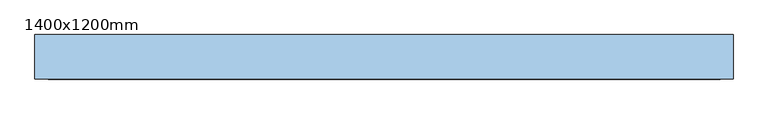
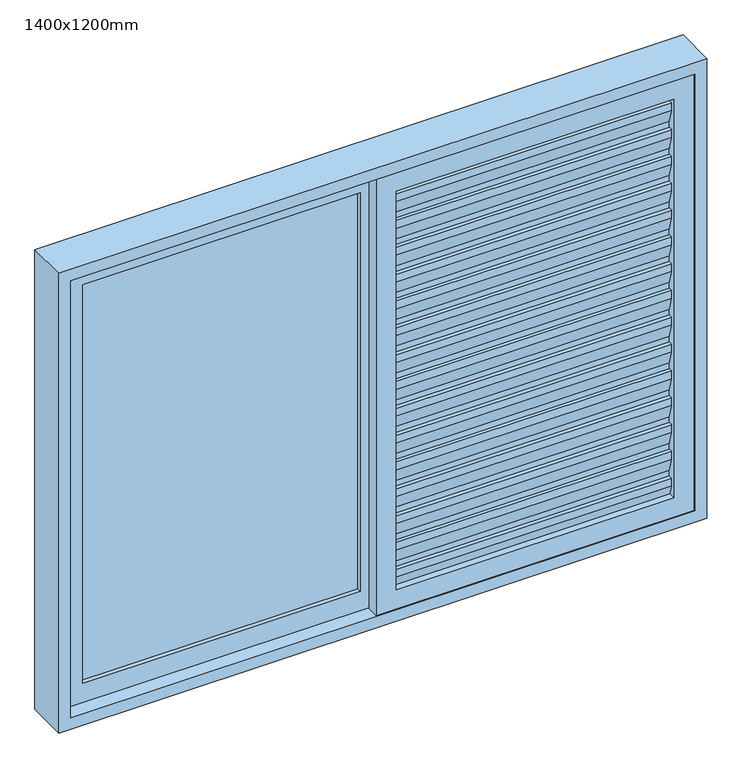
"""IFC4 building model written with IfcOpenShell, lengths in millimetres: window geometry, Janela Veneziana de Correr - 3 Folhas : 1400x1200mm."""

from ifc_helpers import new_model, si_unit, frame, origin, place, context, project, spatial, polyline, outline, extrude, source, transform, mapped, element, save


def window_1400x1200mm_c109a5c7(model_context):
    return source(origin(), model_context, "Body", "SweptSolid", [
        extrude(outline(polyline([(-6.6, 1125.0), (3.4, 1125.0), (3.4, 1140.0), (-6.6, 1175.0), (-6.6, 1195.0), (3.4, 1195.0), (3.4, 1210.0), (-6.6, 1245.0), (-6.6, 1265.0), (3.4, 1265.0), (3.4, 1280.0), (-6.6, 1315.0), (-6.6, 1335.0), (3.4, 1335.0), (3.4, 1350.0), (-6.6, 1385.0), (-6.6, 1405.0), (3.4, 1405.0), (3.4, 1420.0), (-6.6, 1455.0), (-6.6, 1475.0), (3.4, 1475.0), (3.4, 1490.0), (-6.6, 1525.0), (-6.6, 1545.0), (3.4, 1545.0), (3.4, 1560.0), (-6.6, 1595.0), (-6.6, 1615.0), (3.4, 1615.0), (3.4, 1630.0), (-6.6, 1665.0), (-6.6, 1685.0), (3.4, 1685.0), (3.4, 1700.0), (-6.6, 1735.0), (-6.6, 1755.0), (3.4, 1755.0), (3.4, 1770.0), (-6.6, 1805.0), (-6.6, 1825.0), (3.4, 1825.0), (3.4, 1840.0), (-6.6, 1875.0), (-6.6, 1895.0), (3.4, 1895.0), (3.4, 1910.0), (-6.6, 1945.0), (-6.6, 1965.0), (3.4, 1965.0), (3.4, 1980.0), (-6.6, 2015.0), (-6.6, 2035.0), (3.4, 2035.0), (3.4, 2050.0), (-6.6, 2085.0), (-6.6, 2105.0), (3.4, 2105.0), (3.4, 2120.0), (4.4, 2120.1400549), (4.4, 2104.0), (-5.6, 2104.0), (-5.6, 2085.1400549), (4.4, 2050.1400549), (4.4, 2034.0), (-5.6, 2034.0), (-5.6, 2015.1400549), (4.4, 1980.1400549), (4.4, 1964.0), (-5.6, 1964.0), (-5.6, 1945.1400549), (4.4, 1910.1400549), (4.4, 1894.0), (-5.6, 1894.0), (-5.6, 1875.1400549), (4.4, 1840.1400549), (4.4, 1824.0), (-5.6, 1824.0), (-5.6, 1805.1400549), (4.4, 1770.1400549), (4.4, 1754.0), (-5.6, 1754.0), (-5.6, 1735.1400549), (4.4, 1700.1400549), (4.4, 1684.0), (-5.6, 1684.0), (-5.6, 1665.1400549), (4.4, 1630.1400549), (4.4, 1614.0), (-5.6, 1614.0), (-5.6, 1595.1400549), (4.4, 1560.1400549), (4.4, 1544.0), (-5.6, 1544.0), (-5.6, 1525.1400549), (4.4, 1490.1400549), (4.4, 1474.0), (-5.6, 1474.0), (-5.6, 1455.1400549), (4.4, 1420.1400549), (4.4, 1404.0), (-5.6, 1404.0), (-5.6, 1385.1400549), (4.4, 1350.1400549), (4.4, 1334.0), (-5.6, 1334.0), (-5.6, 1315.1400549), (4.4, 1280.1400549), (4.4, 1264.0), (-5.6, 1264.0), (-5.6, 1245.1400549), (4.4, 1210.1400549), (4.4, 1194.0), (-5.6, 1194.0), (-5.6, 1175.1400549), (4.4, 1140.1400549), (4.4, 1124.0), (-5.6, 1124.0), (-5.6, 1105.1400549), (1.5428571, 1080.1400549), (0.5028414, 1080.1400549), (-6.6, 1105.0), (-6.6, 1125.0)])), frame((35.0, 0.0, 0.0), z_axis=(1.0, 0.0, 0.0), x_axis=(0.0, 1.0, 0.0)), (0.0, 0.0, 1.0), 685.0),
        extrude(outline(polyline([(-72.6, 1125.0), (-62.6, 1125.0), (-62.6, 1140.0), (-72.6, 1175.0), (-72.6, 1195.0), (-62.6, 1195.0), (-62.6, 1210.0), (-72.6, 1245.0), (-72.6, 1265.0), (-62.6, 1265.0), (-62.6, 1280.0), (-72.6, 1315.0), (-72.6, 1335.0), (-62.6, 1335.0), (-62.6, 1350.0), (-72.6, 1385.0), (-72.6, 1405.0), (-62.6, 1405.0), (-62.6, 1420.0), (-72.6, 1455.0), (-72.6, 1475.0), (-62.6, 1475.0), (-62.6, 1490.0), (-72.6, 1525.0), (-72.6, 1545.0), (-62.6, 1545.0), (-62.6, 1560.0), (-72.6, 1595.0), (-72.6, 1615.0), (-62.6, 1615.0), (-62.6, 1630.0), (-72.6, 1665.0), (-72.6, 1685.0), (-62.6, 1685.0), (-62.6, 1700.0), (-72.6, 1735.0), (-72.6, 1755.0), (-62.6, 1755.0), (-62.6, 1770.0), (-72.6, 1805.0), (-72.6, 1825.0), (-62.6, 1825.0), (-62.6, 1840.0), (-72.6, 1875.0), (-72.6, 1895.0), (-62.6, 1895.0), (-62.6, 1910.0), (-72.6, 1945.0), (-72.6, 1965.0), (-62.6, 1965.0), (-62.6, 1980.0), (-72.6, 2015.0), (-72.6, 2035.0), (-62.6, 2035.0), (-62.6, 2050.0), (-72.6, 2085.0), (-72.6, 2105.0), (-62.6, 2105.0), (-62.6, 2120.0), (-61.6, 2120.1400549), (-61.6, 2104.0), (-71.6, 2104.0), (-71.6, 2085.1400549), (-61.6, 2050.1400549), (-61.6, 2034.0), (-71.6, 2034.0), (-71.6, 2015.1400549), (-61.6, 1980.1400549), (-61.6, 1964.0), (-71.6, 1964.0), (-71.6, 1945.1400549), (-61.6, 1910.1400549), (-61.6, 1894.0), (-71.6, 1894.0), (-71.6, 1875.1400549), (-61.6, 1840.1400549), (-61.6, 1824.0), (-71.6, 1824.0), (-71.6, 1805.1400549), (-61.6, 1770.1400549), (-61.6, 1754.0), (-71.6, 1754.0), (-71.6, 1735.1400549), (-61.6, 1700.1400549), (-61.6, 1684.0), (-71.6, 1684.0), (-71.6, 1665.1400549), (-61.6, 1630.1400549), (-61.6, 1614.0), (-71.6, 1614.0), (-71.6, 1595.1400549), (-61.6, 1560.1400549), (-61.6, 1544.0), (-71.6, 1544.0), (-71.6, 1525.1400549), (-61.6, 1490.1400549), (-61.6, 1474.0), (-71.6, 1474.0), (-71.6, 1455.1400549), (-61.6, 1420.1400549), (-61.6, 1404.0), (-71.6, 1404.0), (-71.6, 1385.1400549), (-61.6, 1350.1400549), (-61.6, 1334.0), (-71.6, 1334.0), (-71.6, 1315.1400549), (-61.6, 1280.1400549), (-61.6, 1264.0), (-71.6, 1264.0), (-71.6, 1245.1400549), (-61.6, 1210.1400549), (-61.6, 1194.0), (-71.6, 1194.0), (-71.6, 1175.1400549), (-61.6, 1140.1400549), (-61.6, 1124.0), (-71.6, 1124.0), (-71.6, 1105.1400549), (-64.4571429, 1080.1400549), (-65.4971586, 1080.1400549), (-72.6, 1105.0), (-72.6, 1125.0)])), frame((35.0, 0.0, 0.0), z_axis=(1.0, 0.0, 0.0), x_axis=(0.0, 1.0, 0.0)), (0.0, 0.0, 1.0), 685.0),
        extrude(outline(polyline([(2170.0, -15.0), (1030.0, -15.0), (1030.0, 770.0), (2170.0, 770.0), (2170.0, -15.0)]), holes=[polyline([(2120.0, 35.0), (2120.0, 720.0), (1080.0, 720.0), (1080.0, 35.0), (2120.0, 35.0)])]), frame((0.0, -16.6, 0.0), z_axis=(0.0, 1.0, 0.0), x_axis=(0.0, 0.0, 1.0)), (0.0, 0.0, 1.0), 30.0),
        extrude(outline(polyline([(2170.0, -15.0), (1030.0, -15.0), (1030.0, 770.0), (2170.0, 770.0), (2170.0, -15.0)]), holes=[polyline([(2120.0, 35.0), (2120.0, 720.0), (1080.0, 720.0), (1080.0, 35.0), (2120.0, 35.0)])]), frame((0.0, -82.6, 0.0), z_axis=(0.0, 1.0, 0.0), x_axis=(0.0, 0.0, 1.0)), (0.0, 0.0, 1.0), 30.0),
        extrude(outline(polyline([(-720.0, -31.1), (-35.0, -31.1), (-35.0, -38.1), (-720.0, -38.1), (-720.0, -31.1)])), frame((0.0, 0.0, 1080.0), z_axis=(0.0, 0.0, 1.0), x_axis=(1.0, 0.0, 0.0)), (0.0, 0.0, 1.0), 1040.0),
        extrude(outline(polyline([(2170.0, 15.0), (2170.0, -770.0), (1030.0, -770.0), (1030.0, 15.0), (2170.0, 15.0)]), holes=[polyline([(2120.0, -35.0), (1080.0, -35.0), (1080.0, -720.0), (2120.0, -720.0), (2120.0, -35.0)])]), frame((0.0, -49.6, 0.0), z_axis=(0.0, 1.0, 0.0), x_axis=(0.0, 0.0, 1.0)), (0.0, 0.0, 1.0), 30.0),
        extrude(outline(polyline([(2200.0, 800.0), (2200.0, -800.0), (1000.0, -800.0), (1000.0, 800.0), (2200.0, 800.0)]), holes=[polyline([(2170.0, 770.0), (1030.0, 770.0), (1030.0, -770.0), (2170.0, -770.0), (2170.0, 770.0)])]), frame((0.0, -85.6, 0.0), z_axis=(0.0, 1.0, 0.0), x_axis=(0.0, 0.0, 1.0)), (0.0, 0.0, 1.0), 102.0),
    ])


if __name__ == "__main__":
    model = new_model("IFC4")
    model_context = context("Model", 3, world=origin())
    ifc_project = project(units=[si_unit("LENGTHUNIT", "METRE", prefix="MILLI")], contexts=[model_context])
    site = spatial("IfcSite", under=ifc_project)
    building = spatial("IfcBuilding", under=site)
    placement = place(None, origin())
    window_1400x1200mm_shape = window_1400x1200mm_c109a5c7(model_context)
    element("IfcWindow", 1, ObjectType="Janela Veneziana de Correr - 3 Folhas : 1400x1200mm", at=placement, inside=building, context=model_context, shape_type="MappedRepresentation", body=[
        mapped(window_1400x1200mm_shape, transform((0.0, 0.0, 0.0), x_axis=(1.0, 0.0, 0.0), y_axis=(0.0, 1.0, 0.0), z_axis=(0.0, 0.0, 1.0))),
    ])
    save(model, "model.ifc")

# Revit data of these elements
# Type "Janela Veneziana de Correr - 3 Folhas : 1400x1200mm"
#   Type Mark = ""
#   SINAPI = ""
#   Tolerância = 0.30 cm
#   Módulo Básico M = 10.00 cm
#   Largura de Coordenação Modular CM = 160.00 cm
#   Largura Vão = 68.50 cm
#   Largura Veneziana = 69.40 cm
#   Espessura Montante = 3.00 cm
#   Largura Batente = 10.00 cm
#   L_est_v marco = 5.00 cm
#   L_est_h_marco = 5.00 cm
#   L_contramarco = 3.00 cm
#   Altura de Coordenação Modular CM = 120.00 cm
#   Altura Peitoril = 95.00 cm
#   Height = 120.00 cm
#   Width = 160.00 cm
#   Número de Módulos Básicos nM Largura = 16
#   Número de Módulos Básicos nM Altura = 12
#   Material estrutura = Metal - Alumínio
#   Material Quadro = Metal - Alumínio
#   Material Painel = Vidro
#   Type Comments = ""
#   Wall Closure = (empty or 0)
#   Construction Type = (empty or 0)
#   Assembly Code = ""
# Element 1 (IfcWindow, "Janela Veneziana de Correr - 3 Folhas : 1400x1200mm")
#   Materials on its faces: "Metal - Alumínio", "Vidro"
# Materials
#   "Metal - Alumínio": class "Metal", colour RGB 244 244 244, transparency 0
#   "Vidro": class "Vidro", colour RGB 230 230 230, transparency 0.75, Cost = 0
